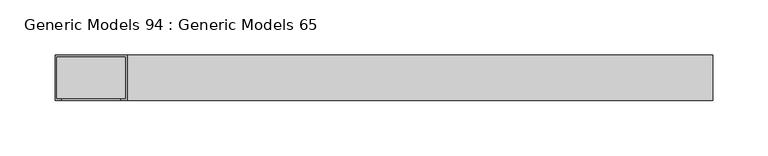
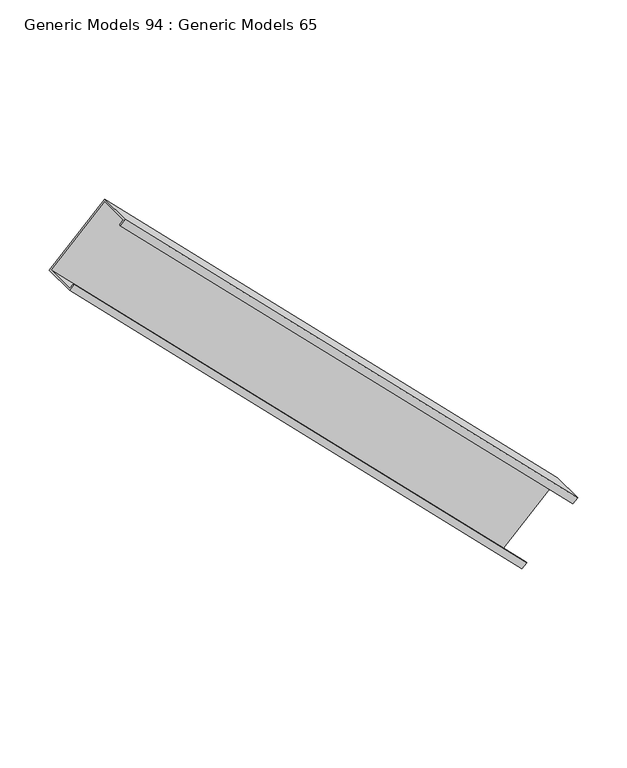
"""IFC4 building model written with IfcOpenShell, lengths in millimetres: proxy geometry, Generic Models 94 : Generic Models 65."""

import ifcopenshell
import ifcopenshell.guid

model = None  # the IFC model being written
_history = None  # IfcOwnerHistory: only IFC2X3 demands one
_inside = {}  # id of a spatial element -> (the spatial element, [elements in it])
_under = {}  # id of a project, library or spatial element -> (it, [spatial elements below it])
_declared = {}  # id of a project -> (the project, [libraries it declares])
_typed = {}  # id of a type object -> (the type object, [elements of that type])
_made_of = {}  # id of a material, layer set ... -> (it, [elements and type objects made of it])


def new_model(schema):
    """Start an empty IFC model of exactly this schema.

    Asked for "IFC4X3", IfcOpenShell would pick the latest addendum, in which some entities
    have other attributes; the version numbers below select the first issue.
    IFC2X3 requires an IfcOwnerHistory on every rooted entity: one is made here for all.
    """
    global model, _history
    if schema == "IFC4X3":
        model = ifcopenshell.file(schema_version=(4, 3, 0, 0))
    else:
        model = ifcopenshell.file(schema=schema)
    _inside.clear()
    _under.clear()
    _declared.clear()
    _typed.clear()
    _made_of.clear()
    _history = None
    if model.schema == "IFC2X3":
        org = make("IfcOrganization", Name="unknown")
        user = make(
            "IfcPersonAndOrganization",
            ThePerson=make("IfcPerson", FamilyName="unknown"),
            TheOrganization=org,
        )
        app = make(
            "IfcApplication",
            ApplicationDeveloper=org,
            Version="unknown",
            ApplicationFullName="unknown",
            ApplicationIdentifier="unknown",
        )
        _history = make(
            "IfcOwnerHistory",
            OwningUser=user,
            OwningApplication=app,
            ChangeAction="ADDED",
            CreationDate=0,
        )
    return model


def make(cls, **values):
    """One entity of the class cls with the attributes given. An attribute that is None is left unset."""
    return model.create_entity(
        cls, **{name: value for name, value in values.items() if value is not None}
    )


def rooted(cls, **values):
    """An entity with a GlobalId (a new one), such as an element, a storey or a relation."""
    return make(cls, GlobalId=ifcopenshell.guid.new(), OwnerHistory=_history, **values)


def si_unit(unit_type, name, prefix=None):
    """IfcSIUnit, for example si_unit("LENGTHUNIT", "METRE", prefix="MILLI")."""
    return make("IfcSIUnit", UnitType=unit_type, Prefix=prefix, Name=name)


def assignment(units):
    """IfcUnitAssignment: the units of a project."""
    return None if units is None else make("IfcUnitAssignment", Units=units)


def point(xyz):
    """IfcCartesianPoint."""
    return None if xyz is None else make("IfcCartesianPoint", Coordinates=xyz)


def direction(xyz):
    """IfcDirection."""
    return None if xyz is None else make("IfcDirection", DirectionRatios=xyz)


def frame(location, z_axis=None, x_axis=None):
    """IfcAxis2Placement3D, a coordinate frame: its origin and axes. An axis left out is left unset."""
    return make(
        "IfcAxis2Placement3D",
        Location=point(location),
        Axis=direction(z_axis),
        RefDirection=direction(x_axis),
    )


def origin():
    """The frame at (0, 0, 0) with its axes left unset."""
    return frame((0.0, 0.0, 0.0))


def place(relative_to, where):
    """IfcLocalPlacement: puts the frame where relative to a parent placement (None: the world)."""
    return make(
        "IfcLocalPlacement", PlacementRelTo=relative_to, RelativePlacement=where
    )


def context(
    kind, dimensions, precision=None, world=None, true_north=None, identifier=None
):
    """IfcGeometricRepresentationContext, for example the 3D "Model" context."""
    return make(
        "IfcGeometricRepresentationContext",
        ContextIdentifier=identifier,
        ContextType=kind,
        CoordinateSpaceDimension=dimensions,
        Precision=precision,
        WorldCoordinateSystem=world,
        TrueNorth=true_north,
    )


def project(units=None, contexts=None):
    """IfcProject with its units and contexts."""
    return rooted(
        "IfcProject",
        Name="project",
        RepresentationContexts=contexts,
        UnitsInContext=assignment(units),
    )


def spatial(cls, under=None, at=None, **own):
    """A site, building, storey or space (cls), placed at a placement, below another one or the project."""
    s = rooted(cls, ObjectPlacement=at, **own)
    if under is not None:
        _under.setdefault(under.id(), (under, []))[1].append(s)
    return s


def polyline(points):
    """IfcPolyline through the points."""
    return make("IfcPolyline", Points=[point(p) for p in points])


def outline(outer, holes=None, kind="AREA"):
    """IfcArbitraryClosedProfileDef: a profile drawn as a closed curve; with holes, ...WithVoids."""
    if holes is None:
        return make("IfcArbitraryClosedProfileDef", ProfileType=kind, OuterCurve=outer)
    return make(
        "IfcArbitraryProfileDefWithVoids",
        ProfileType=kind,
        OuterCurve=outer,
        InnerCurves=holes,
    )


def extrude(swept, where, along, depth):
    """IfcExtrudedAreaSolid: the profile swept, set in the frame where, extruded along a direction by depth."""
    return make(
        "IfcExtrudedAreaSolid",
        SweptArea=swept,
        Position=where,
        ExtrudedDirection=direction(along),
        Depth=depth,
    )


def shape(context_of_items, identifier, shape_type, items):
    """IfcShapeRepresentation: the items that make up one representation, for example the "Body"."""
    return make(
        "IfcShapeRepresentation",
        ContextOfItems=context_of_items,
        RepresentationIdentifier=identifier,
        RepresentationType=shape_type,
        Items=items,
    )


def source(mapping_origin, context_of_items, identifier, shape_type, items):
    """IfcRepresentationMap: a shape defined once, which mapped items show again and again."""
    return make(
        "IfcRepresentationMap",
        MappingOrigin=mapping_origin,
        MappedRepresentation=shape(context_of_items, identifier, shape_type, items),
    )


def transform(
    local_origin,
    x_axis=None,
    y_axis=None,
    z_axis=None,
    scale=None,
    scale2=None,
    scale3=None,
    uniform=True,
):
    """IfcCartesianTransformationOperator3D, or its non-uniform kind. x_axis, y_axis, z_axis: its Axis1, 2, 3."""
    if uniform:
        return make(
            "IfcCartesianTransformationOperator3D",
            Axis1=direction(x_axis),
            Axis2=direction(y_axis),
            LocalOrigin=point(local_origin),
            Scale=scale,
            Axis3=direction(z_axis),
        )
    return make(
        "IfcCartesianTransformationOperator3DnonUniform",
        Axis1=direction(x_axis),
        Axis2=direction(y_axis),
        LocalOrigin=point(local_origin),
        Scale=scale,
        Axis3=direction(z_axis),
        Scale2=scale2,
        Scale3=scale3,
    )


def mapped(mapping_source, mapping_target):
    """IfcMappedItem: shows the shape of a source again, moved by a transform."""
    return make(
        "IfcMappedItem", MappingSource=mapping_source, MappingTarget=mapping_target
    )


def made_of(thing, what):
    """Note that an element or type object is made of a material, layer set ...; save() writes the relation."""
    if what is not None:
        _made_of.setdefault(what.id(), (what, []))[1].append(thing)
    return thing


def element(
    cls,
    number,
    at=None,
    inside=None,
    cuts=None,
    type_object=None,
    material=None,
    context=None,
    identifier="Body",
    shape_type=None,
    held_by="IfcProductDefinitionShape",
    body=None,
    shapes=None,
    **own,
):
    """One element of the class cls, such as IfcWall. Its Tag is "e" and its number.

    at: its placement. inside: the storey or other place that contains it. cuts: it is an
    opening in that element (IfcRelVoidsElement). A single representation is given by context,
    identifier, shape_type and body (its items); several are given by shapes. held_by: the class
    of the entity that holds the representations. save() writes the other relations.
    """
    e = rooted(cls, Tag="e%d" % number, ObjectPlacement=at, **own)
    if body is not None:
        shapes = [shape(context, identifier, shape_type, body)]
    if shapes is not None:
        e.Representation = make(held_by, Representations=shapes)
    if inside is not None:
        _inside.setdefault(inside.id(), (inside, []))[1].append(e)
    if cuts is not None:
        rooted(
            "IfcRelVoidsElement", RelatingBuildingElement=cuts, RelatedOpeningElement=e
        )
    if type_object is not None:
        _typed.setdefault(type_object.id(), (type_object, []))[1].append(e)
    return made_of(e, material)


def aggregate(whole, parts):
    """IfcRelAggregates: a whole, such as a stair, and the parts it consists of."""
    return rooted("IfcRelAggregates", RelatingObject=whole, RelatedObjects=parts)


def save(model, path):
    """Write the relations noted so far, then the file.

    IfcRelAggregates (storeys below a building ...), IfcRelContainedInSpatialStructure (elements
    in a storey), IfcRelDefinesByType, IfcRelAssociatesMaterial and IfcRelDeclares: one each for
    every whole, place, type object, material and project.
    """
    for whole, parts in _under.values():
        aggregate(whole, parts)
    for where, things in _inside.values():
        rooted(
            "IfcRelContainedInSpatialStructure",
            RelatedElements=things,
            RelatingStructure=where,
        )
    for kind, things in _typed.values():
        rooted("IfcRelDefinesByType", RelatedObjects=things, RelatingType=kind)
    for what, things in _made_of.values():
        rooted("IfcRelAssociatesMaterial", RelatedObjects=things, RelatingMaterial=what)
    for by, libraries in _declared.values():
        rooted("IfcRelDeclares", RelatingContext=by, RelatedDefinitions=libraries)
    model.write(path)


def generic_models_94_generic_models_65_e95720d5(model_context):
    return source(origin(), model_context, "Body", "SweptSolid", [
        extrude(outline(polyline([(0.0, -92.075), (0.0, 0.0), (41.275, 0.0), (41.275, -7.9375), (39.6875, -7.9375), (39.6875, -1.5875), (1.5875, -1.5875), (1.5875, -90.4875001), (39.6875, -90.4875001), (39.6875, -84.1375), (41.275, -84.1375), (41.275, -92.075), (0.0, -92.075)])), frame((48147.1360531, 630.2375, 1792.900826), z_axis=(-0.7071067811865384, 0.0, 0.7071067811865568), x_axis=(0.0, -1.0, 0.0)), (0.0, 0.0, 1.0), 749.9641452),
    ])


if __name__ == "__main__":
    model = new_model("IFC4")
    model_context = context("Model", 3, world=origin())
    ifc_project = project(units=[si_unit("LENGTHUNIT", "METRE", prefix="MILLI")], contexts=[model_context])
    site = spatial("IfcSite", under=ifc_project)
    building = spatial("IfcBuilding", under=site)
    placement = place(None, origin())
    generic_models_94_generic_models_65_shape = generic_models_94_generic_models_65_e95720d5(model_context)
    element("IfcBuildingElementProxy", 1, Name="Generic Models 94 : Generic Models 65", ObjectType="Generic Models 94 : Generic Models 65", at=placement, inside=building, context=model_context, shape_type="MappedRepresentation", body=[
        mapped(generic_models_94_generic_models_65_shape, transform((0.0, 0.0, 0.0), x_axis=(1.0, 0.0, 0.0), y_axis=(0.0, 1.0, 0.0), z_axis=(0.0, 0.0, 1.0))),
    ])
    save(model, "model.ifc")

# Revit data of these elements
# Element 1 (IfcBuildingElementProxy, "Generic Models 94 : Generic Models 65")
#   Materials on its faces: "DIAGONAL BRACING AS NECESSARY - ATTACH TO STRUCTURAL DECK"
# Materials
#   "DIAGONAL BRACING AS NECESSARY - ATTACH TO STRUCTURAL DECK": class "Unassigned", colour RGB 210 209 208, transparency 0, Keynote = "M05121300.02", Cost = 0
